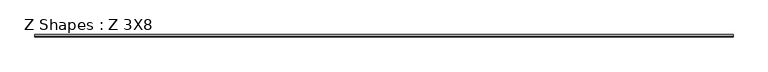
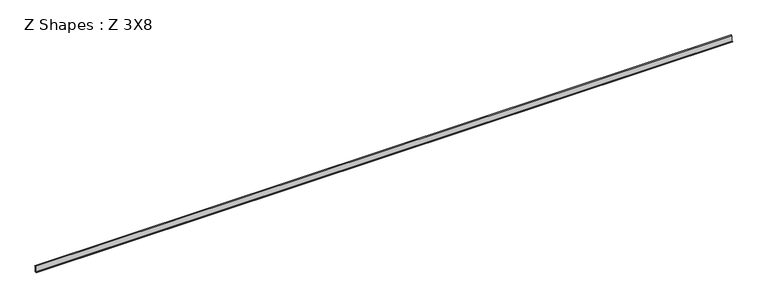
"""IFC4 building model written with IfcOpenShell, lengths in millimetres: beam geometry, Z Shapes : Z 3X8."""

import ifcopenshell
import ifcopenshell.guid

model = None  # the IFC model being written
_history = None  # IfcOwnerHistory: only IFC2X3 demands one
_inside = {}  # id of a spatial element -> (the spatial element, [elements in it])
_under = {}  # id of a project, library or spatial element -> (it, [spatial elements below it])
_declared = {}  # id of a project -> (the project, [libraries it declares])
_typed = {}  # id of a type object -> (the type object, [elements of that type])
_made_of = {}  # id of a material, layer set ... -> (it, [elements and type objects made of it])


def new_model(schema):
    """Start an empty IFC model of exactly this schema.

    Asked for "IFC4X3", IfcOpenShell would pick the latest addendum, in which some entities
    have other attributes; the version numbers below select the first issue.
    IFC2X3 requires an IfcOwnerHistory on every rooted entity: one is made here for all.
    """
    global model, _history
    if schema == "IFC4X3":
        model = ifcopenshell.file(schema_version=(4, 3, 0, 0))
    else:
        model = ifcopenshell.file(schema=schema)
    _inside.clear()
    _under.clear()
    _declared.clear()
    _typed.clear()
    _made_of.clear()
    _history = None
    if model.schema == "IFC2X3":
        org = make("IfcOrganization", Name="unknown")
        user = make(
            "IfcPersonAndOrganization",
            ThePerson=make("IfcPerson", FamilyName="unknown"),
            TheOrganization=org,
        )
        app = make(
            "IfcApplication",
            ApplicationDeveloper=org,
            Version="unknown",
            ApplicationFullName="unknown",
            ApplicationIdentifier="unknown",
        )
        _history = make(
            "IfcOwnerHistory",
            OwningUser=user,
            OwningApplication=app,
            ChangeAction="ADDED",
            CreationDate=0,
        )
    return model


def make(cls, **values):
    """One entity of the class cls with the attributes given. An attribute that is None is left unset."""
    return model.create_entity(
        cls, **{name: value for name, value in values.items() if value is not None}
    )


def rooted(cls, **values):
    """An entity with a GlobalId (a new one), such as an element, a storey or a relation."""
    return make(cls, GlobalId=ifcopenshell.guid.new(), OwnerHistory=_history, **values)


def si_unit(unit_type, name, prefix=None):
    """IfcSIUnit, for example si_unit("LENGTHUNIT", "METRE", prefix="MILLI")."""
    return make("IfcSIUnit", UnitType=unit_type, Prefix=prefix, Name=name)


def assignment(units):
    """IfcUnitAssignment: the units of a project."""
    return None if units is None else make("IfcUnitAssignment", Units=units)


def point(xyz):
    """IfcCartesianPoint."""
    return None if xyz is None else make("IfcCartesianPoint", Coordinates=xyz)


def direction(xyz):
    """IfcDirection."""
    return None if xyz is None else make("IfcDirection", DirectionRatios=xyz)


def frame(location, z_axis=None, x_axis=None):
    """IfcAxis2Placement3D, a coordinate frame: its origin and axes. An axis left out is left unset."""
    return make(
        "IfcAxis2Placement3D",
        Location=point(location),
        Axis=direction(z_axis),
        RefDirection=direction(x_axis),
    )


def origin():
    """The frame at (0, 0, 0) with its axes left unset."""
    return frame((0.0, 0.0, 0.0))


def place(relative_to, where):
    """IfcLocalPlacement: puts the frame where relative to a parent placement (None: the world)."""
    return make(
        "IfcLocalPlacement", PlacementRelTo=relative_to, RelativePlacement=where
    )


def context(
    kind, dimensions, precision=None, world=None, true_north=None, identifier=None
):
    """IfcGeometricRepresentationContext, for example the 3D "Model" context."""
    return make(
        "IfcGeometricRepresentationContext",
        ContextIdentifier=identifier,
        ContextType=kind,
        CoordinateSpaceDimension=dimensions,
        Precision=precision,
        WorldCoordinateSystem=world,
        TrueNorth=true_north,
    )


def project(units=None, contexts=None):
    """IfcProject with its units and contexts."""
    return rooted(
        "IfcProject",
        Name="project",
        RepresentationContexts=contexts,
        UnitsInContext=assignment(units),
    )


def spatial(cls, under=None, at=None, **own):
    """A site, building, storey or space (cls), placed at a placement, below another one or the project."""
    s = rooted(cls, ObjectPlacement=at, **own)
    if under is not None:
        _under.setdefault(under.id(), (under, []))[1].append(s)
    return s


def polyline(points):
    """IfcPolyline through the points."""
    return make("IfcPolyline", Points=[point(p) for p in points])


def outline(outer, holes=None, kind="AREA"):
    """IfcArbitraryClosedProfileDef: a profile drawn as a closed curve; with holes, ...WithVoids."""
    if holes is None:
        return make("IfcArbitraryClosedProfileDef", ProfileType=kind, OuterCurve=outer)
    return make(
        "IfcArbitraryProfileDefWithVoids",
        ProfileType=kind,
        OuterCurve=outer,
        InnerCurves=holes,
    )


def extrude(swept, where, along, depth):
    """IfcExtrudedAreaSolid: the profile swept, set in the frame where, extruded along a direction by depth."""
    return make(
        "IfcExtrudedAreaSolid",
        SweptArea=swept,
        Position=where,
        ExtrudedDirection=direction(along),
        Depth=depth,
    )


def shape(context_of_items, identifier, shape_type, items):
    """IfcShapeRepresentation: the items that make up one representation, for example the "Body"."""
    return make(
        "IfcShapeRepresentation",
        ContextOfItems=context_of_items,
        RepresentationIdentifier=identifier,
        RepresentationType=shape_type,
        Items=items,
    )


def source(mapping_origin, context_of_items, identifier, shape_type, items):
    """IfcRepresentationMap: a shape defined once, which mapped items show again and again."""
    return make(
        "IfcRepresentationMap",
        MappingOrigin=mapping_origin,
        MappedRepresentation=shape(context_of_items, identifier, shape_type, items),
    )


def transform(
    local_origin,
    x_axis=None,
    y_axis=None,
    z_axis=None,
    scale=None,
    scale2=None,
    scale3=None,
    uniform=True,
):
    """IfcCartesianTransformationOperator3D, or its non-uniform kind. x_axis, y_axis, z_axis: its Axis1, 2, 3."""
    if uniform:
        return make(
            "IfcCartesianTransformationOperator3D",
            Axis1=direction(x_axis),
            Axis2=direction(y_axis),
            LocalOrigin=point(local_origin),
            Scale=scale,
            Axis3=direction(z_axis),
        )
    return make(
        "IfcCartesianTransformationOperator3DnonUniform",
        Axis1=direction(x_axis),
        Axis2=direction(y_axis),
        LocalOrigin=point(local_origin),
        Scale=scale,
        Axis3=direction(z_axis),
        Scale2=scale2,
        Scale3=scale3,
    )


def mapped(mapping_source, mapping_target):
    """IfcMappedItem: shows the shape of a source again, moved by a transform."""
    return make(
        "IfcMappedItem", MappingSource=mapping_source, MappingTarget=mapping_target
    )


def made_of(thing, what):
    """Note that an element or type object is made of a material, layer set ...; save() writes the relation."""
    if what is not None:
        _made_of.setdefault(what.id(), (what, []))[1].append(thing)
    return thing


def element(
    cls,
    number,
    at=None,
    inside=None,
    cuts=None,
    type_object=None,
    material=None,
    context=None,
    identifier="Body",
    shape_type=None,
    held_by="IfcProductDefinitionShape",
    body=None,
    shapes=None,
    **own,
):
    """One element of the class cls, such as IfcWall. Its Tag is "e" and its number.

    at: its placement. inside: the storey or other place that contains it. cuts: it is an
    opening in that element (IfcRelVoidsElement). A single representation is given by context,
    identifier, shape_type and body (its items); several are given by shapes. held_by: the class
    of the entity that holds the representations. save() writes the other relations.
    """
    e = rooted(cls, Tag="e%d" % number, ObjectPlacement=at, **own)
    if body is not None:
        shapes = [shape(context, identifier, shape_type, body)]
    if shapes is not None:
        e.Representation = make(held_by, Representations=shapes)
    if inside is not None:
        _inside.setdefault(inside.id(), (inside, []))[1].append(e)
    if cuts is not None:
        rooted(
            "IfcRelVoidsElement", RelatingBuildingElement=cuts, RelatedOpeningElement=e
        )
    if type_object is not None:
        _typed.setdefault(type_object.id(), (type_object, []))[1].append(e)
    return made_of(e, material)


def aggregate(whole, parts):
    """IfcRelAggregates: a whole, such as a stair, and the parts it consists of."""
    return rooted("IfcRelAggregates", RelatingObject=whole, RelatedObjects=parts)


def save(model, path):
    """Write the relations noted so far, then the file.

    IfcRelAggregates (storeys below a building ...), IfcRelContainedInSpatialStructure (elements
    in a storey), IfcRelDefinesByType, IfcRelAssociatesMaterial and IfcRelDeclares: one each for
    every whole, place, type object, material and project.
    """
    for whole, parts in _under.values():
        aggregate(whole, parts)
    for where, things in _inside.values():
        rooted(
            "IfcRelContainedInSpatialStructure",
            RelatedElements=things,
            RelatingStructure=where,
        )
    for kind, things in _typed.values():
        rooted("IfcRelDefinesByType", RelatedObjects=things, RelatingType=kind)
    for what, things in _made_of.values():
        rooted("IfcRelAssociatesMaterial", RelatedObjects=things, RelatingMaterial=what)
    for by, libraries in _declared.values():
        rooted("IfcRelDeclares", RelatingContext=by, RelatedDefinitions=libraries)
    model.write(path)


def z_shapes_z_3x8_f6795473(model_context):
    return source(origin(), model_context, "Body", "SweptSolid", [
        extrude(outline(polyline([(57.2805719, 92.452825), (27.1991352, 92.452825), (27.1991352, -98.809175), (-18.9194281, -98.809175), (-18.9194281, -92.459175), (19.1805719, -92.459175), (19.1805719, 102.104825), (57.2805719, 102.104825), (57.2805719, 92.452825)])), frame((-11474.45, 0.0, 0.0), z_axis=(1.0, 0.0, 0.0), x_axis=(0.0, 1.0, 0.0)), (0.0, 0.0, 1.0), 23361.65),
    ])


if __name__ == "__main__":
    model = new_model("IFC4")
    model_context = context("Model", 3, world=origin())
    ifc_project = project(units=[si_unit("LENGTHUNIT", "METRE", prefix="MILLI")], contexts=[model_context])
    site = spatial("IfcSite", under=ifc_project)
    building = spatial("IfcBuilding", under=site)
    placement = place(None, origin())
    z_shapes_z_3x8_shape = z_shapes_z_3x8_f6795473(model_context)
    element("IfcBeam", 1, ObjectType="Z Shapes : Z 3X8", at=placement, inside=building, context=model_context, shape_type="MappedRepresentation", body=[
        mapped(z_shapes_z_3x8_shape, transform((0.0, 0.0, 0.0), x_axis=(1.0, 0.0, 0.0), y_axis=(0.0, 1.0, 0.0), z_axis=(0.0, 0.0, 1.0))),
    ])
    save(model, "model.ifc")

# Revit data of these elements
# Type "Z Shapes : Z 3X8"
#   Section Name Key = "W12x26"
#   Assembly Code = "B10"
#   Width = 76.2 mm
#   Web Thickness = 5.842 mm
#   Web Fillet = 7.62 mm
#   Warping Constant = 163001.3 cm⁶
#   Torsional Moment of Inertia = 12.4869 cm⁴
#   Section Area = 7.65 in²
#   Plastic Modulus weak axis = 0.00472801 (stored number, unit not read)
#   Plastic Modulus strong axis = 0.0215278 (stored number, unit not read)
#   Perimeter = 15.0571 m²/m
#   Nominal Weight = 379.441 N/m
#   Moment of Inertia weak axis = 720.08 cm⁴
#   Moment of Inertia strong axis = 8491.12 cm⁴
#   Height = 184.912 mm
#   Flange Thickness = 9.652 mm
#   Elastic Modulus weak axis = 0.00309028 (stored number, unit not read)
#   Elastic Modulus strong axis = 0.0193287 (stored number, unit not read)
#   Centroid Vertical = 92.456 mm
#   Centroid Horizontal = 38.1 mm
#   Length [instance default] = 5' - 0"
#   Structural Material [instance default] = Steel ASTM A992
#   Principal Axes Angle = 0
# Element 1 (IfcBeam, "Z Shapes : Z 3X8")
#   Materials on its faces: "Steel ASTM A992"
# Materials
#   "Steel ASTM A992": class "Metal", colour RGB 189 187 185, transparency 0, Description = "Structural steel 50ksi", Cost = 0
